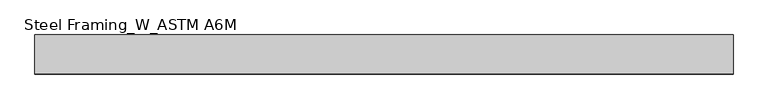
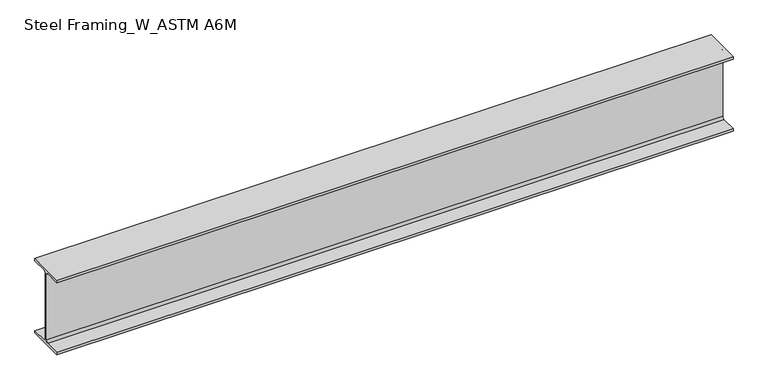
"""IFC4 building model written with IfcOpenShell, lengths in millimetres: beam geometry, Steel Framing_W_ASTM A6M : H_SB_AR_S02_W360x51_G3."""

from ifc_helpers import new_model, si_unit, point, frame, frame_2d, origin, place, context, project, spatial, polyline, circle_curve, trimmed, segment, composite_curve, outline, extrude, source, transform, mapped, element, save


def steel_framing_w_astm_a6m_38a99291(model_context):
    return source(origin(), model_context, "Body", "SweptSolid", [
        extrude(outline(composite_curve([segment(polyline([(85.5, -166.4), (85.5, -178.0), (-85.5, -178.0), (-85.5, -166.4), (-13.72, -166.4)]), True, "CONTINUOUS"), segment(trimmed(circle_curve(frame_2d((-13.72, -156.3)), 10.1), [point((-13.72, -166.4))], [point((-3.62, -156.3))], True, "CARTESIAN"), True, "CONTINUOUS"), segment(polyline([(-3.62, -156.3), (-3.62, 156.3)]), True, "CONTINUOUS"), segment(trimmed(circle_curve(frame_2d((-13.72, 156.3)), 10.1), [point((-3.62, 156.3))], [point((-13.72, 166.4))], True, "CARTESIAN"), True, "CONTINUOUS"), segment(polyline([(-13.72, 166.4), (-85.5, 166.4), (-85.5, 178.0), (85.5, 178.0), (85.5, 166.4), (13.72, 166.4)]), True, "CONTINUOUS"), segment(trimmed(circle_curve(frame_2d((13.72, 156.3)), 10.1), [point((13.72, 166.4))], [point((3.62, 156.3))], True, "CARTESIAN"), True, "CONTINUOUS"), segment(polyline([(3.62, 156.3), (3.62, -156.3)]), True, "CONTINUOUS"), segment(trimmed(circle_curve(frame_2d((13.72, -156.3)), 10.1), [point((3.62, -156.3))], [point((13.72, -166.4))], True, "CARTESIAN"), True, "CONTINUOUS"), segment(polyline([(13.72, -166.4), (85.5, -166.4)]), True, "CONTINUOUS")], self_intersect=False)), frame((-1487.2, 0.0, 0.0), z_axis=(1.0, 0.0, 0.0), x_axis=(0.0, 1.0, 0.0)), (0.0, 0.0, 1.0), 3054.2),
    ])


if __name__ == "__main__":
    model = new_model("IFC4")
    model_context = context("Model", 3, world=origin())
    ifc_project = project(units=[si_unit("LENGTHUNIT", "METRE", prefix="MILLI")], contexts=[model_context])
    site = spatial("IfcSite", under=ifc_project)
    building = spatial("IfcBuilding", under=site)
    placement = place(None, origin())
    steel_framing_w_astm_a6m_shape = steel_framing_w_astm_a6m_38a99291(model_context)
    element("IfcBeam", 1, ObjectType="Steel Framing_W_ASTM A6M : H_SB_AR_S02_W360x51_G3", at=placement, inside=building, context=model_context, shape_type="MappedRepresentation", body=[
        mapped(steel_framing_w_astm_a6m_shape, transform((0.0, 0.0, 0.0), x_axis=(1.0, 0.0, 0.0), y_axis=(0.0, 1.0, 0.0), z_axis=(0.0, 0.0, 1.0))),
    ])
    save(model, "model.ifc")

# Revit data of these elements
# Type "Steel Framing_W_ASTM A6M : H_SB_AR_S02_W360x51_G3"
#   Type Mark = "G3"
#   Section Name Key = "W14x34"
#   Width = 17.1 cm
#   Web Thickness = 0.724 cm
#   Web Fillet = 1.01 cm
#   Warping Constant = 287000.0 cm⁶
#   Torsional Moment of Inertia = 23.70 cm⁴
#   Section Area = 64.5 cm²
#   Plastic Modulus weak axis = 174.0 cm³
#   Plastic Modulus strong axis = 895.0 cm³
#   Perimeter = 1.36 m²/m
#   Nominal Weight = 51.00 kgf/m
#   Moment of Inertia weak axis = 970.00 cm⁴
#   Moment of Inertia strong axis = 14200.00 cm⁴
#   Height = 35.6 cm
#   Flange Thickness = 1.16 cm
#   Elastic Modulus weak axis = 113.0 cm³
#   Elastic Modulus strong axis = 796.0 cm³
#   Centroid Vertical = 17.8 cm
#   Centroid Horizontal = 8.55 cm
#   Length [instance default] = 1500 mm
#   Structural Material [instance default] = Steel, 45-345
#   Bolt Spacing = 0
#   Assembly Code = ""
# Element 1 (IfcBeam, "Steel Framing_W_ASTM A6M : H_SB_AR_S02_W360x51_G3")
#   Materials on its faces: "Steel, 45-345"
# Materials
#   "Steel, 45-345": class "Metal", colour RGB 189 187 185, transparency 0, Description = "Steel 345 MPa", Cost = 0
